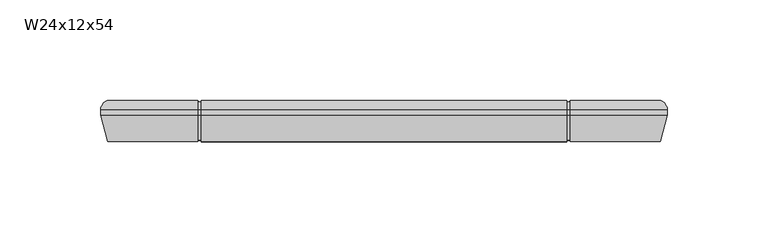
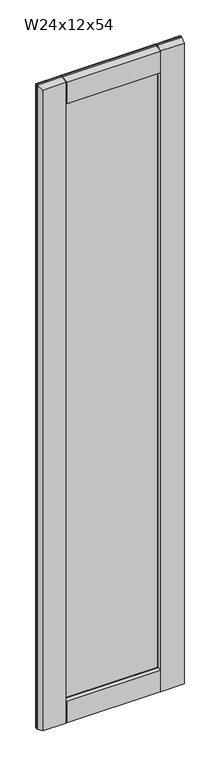
"""IFC4 building model written with IfcOpenShell, lengths in millimetres: furniture geometry, Cabinet-Wall-Merillat-Double_Door-Marlin : W24x12x54."""

from ifc_helpers import new_model, si_unit, frame, origin, place, context, project, spatial, polyline, circle_curve, ellipse_curve, outline, extrude, source, transform, mapped, element, save
from ifc_brep_helpers import plane_surface, cylinder_surface, advanced_brep


def w24x12x54_5feed744(model_context):
    return source(origin(), model_context, "Body", "SolidModel", [
        advanced_brep(
        [(541.0528392, 401.6121, 2108.2), (541.0528392, 401.6121, 787.4), (537.9563467, 406.0825, 790.4964925), (537.9563467, 406.0825, 2105.1035075), (541.0528392, 398.8435, 2108.2), (541.0528392, 398.8435, 787.4), (537.5476392, 385.7625, 2104.6948), (537.5476392, 385.7625, 790.9052), (492.8516765, 385.7625, 2059.9988372), (492.4815448, 386.55625, 2059.6287055), (490.4003857, 391.01931, 2057.5475465), (490.4003857, 391.01931, 838.0524535), (492.4815448, 386.55625, 835.9712945), (492.8516765, 385.7625, 835.6011628), (491.8001552, 393.2594093, 2058.947316), (491.8001552, 393.2594093, 836.652684), (506.1278392, 393.5095, 2073.275), (506.1278392, 393.5095, 822.325), (506.1278392, 398.3355, 2073.275), (506.1278392, 398.3355, 822.325), (491.8001552, 398.5855907, 2058.947316), (491.8001552, 398.5855907, 836.652684), (490.4003857, 400.82569, 2057.5475465), (490.4003857, 400.82569, 838.0524535), (492.4815448, 405.28875, 2059.6287055), (492.848809, 406.0763508, 2059.9959698), (492.8516765, 406.0825, 835.6011628), (492.4815448, 405.28875, 835.9712945), (263.1618317, 406.0825, 790.4964925), (308.2295579, 406.0825, 790.4964925), (308.2295579, 401.6121, 787.4), (260.0653392, 401.6121, 787.4), (492.848809, 401.6121, 787.4), (492.848809, 406.0825, 790.4964925), (491.261309, 401.6121, 787.4), (309.8170579, 401.6121, 787.4), (309.8170579, 406.0825, 790.4964925), (491.261309, 406.0825, 790.4964925), (308.2295579, 398.8435, 787.4), (260.0653392, 398.8435, 787.4), (492.848809, 398.8435, 787.4), (491.261309, 398.8435, 787.4), (309.8170579, 398.8435, 787.4), (308.2295579, 385.7625, 790.9052), (263.5705392, 385.7625, 790.9052), (491.261309, 385.7625, 790.9052), (309.8170579, 385.7625, 790.9052), (492.848809, 385.7625, 790.9052), (310.7177927, 391.01931, 838.0524535), (308.6366337, 386.55625, 835.9712945), (309.8170579, 386.55625, 835.9712945), (309.8170579, 385.7625, 835.6011628), (491.261309, 385.7625, 835.6011628), (491.261309, 386.55625, 835.9712945), (309.3180233, 393.2594093, 836.652684), (294.9903392, 393.5095, 822.325), (294.9903392, 398.3355, 822.325), (309.3180233, 398.5855907, 836.652684), (310.7177927, 400.82569, 838.0524535), (491.261309, 405.28875, 835.9712945), (491.261309, 406.0825, 835.6011628), (309.8170579, 406.0825, 835.6011628), (309.8170579, 405.28875, 835.9712945), (308.6366337, 405.28875, 835.9712945), (260.0653392, 401.6121, 2108.2), (263.1618317, 406.0825, 2105.1035075), (260.0653392, 398.8435, 2108.2), (263.5705392, 385.7625, 2104.6948), (308.266502, 385.7625, 835.6011628), (310.7177927, 391.01931, 2057.5475465), (308.6366337, 386.55625, 2059.6287055), (308.266502, 385.7625, 2059.9988372), (309.3180233, 393.2594093, 2058.947316), (294.9903392, 393.5095, 2073.275), (294.9903392, 398.3355, 2073.275), (309.3180233, 398.5855907, 2058.947316), (310.7177927, 400.82569, 2057.5475465), (308.266502, 406.0825, 835.6011628), (308.266502, 406.0825, 2059.9988372), (308.6366337, 405.28875, 2059.6287055), (492.848809, 406.0825, 2105.1035075), (492.848809, 401.6121, 2108.2), (308.2295579, 401.6121, 2108.2), (308.2295579, 406.0825, 2105.1035075), (309.8170579, 401.6121, 2108.2), (491.261309, 401.6121, 2108.2), (491.261309, 406.0825, 2105.1035075), (309.8170579, 406.0825, 2105.1035075), (492.848809, 398.8435, 2108.2), (308.2295579, 398.8435, 2108.2), (309.8170579, 398.8435, 2108.2), (491.261309, 398.8435, 2108.2), (492.848809, 385.7625, 2104.6948), (308.2295579, 385.7625, 2104.6948), (309.8170579, 385.7625, 2104.6948), (491.261309, 385.7625, 2104.6948), (309.8170579, 385.7625, 2059.9988372), (491.261309, 385.7625, 2059.9988372), (491.261309, 386.55625, 2059.6287055), (309.8170579, 386.55625, 2059.6287055), (309.8170579, 405.28875, 2059.6287055), (309.8170579, 406.0825, 2059.9988372), (491.261309, 406.0825, 2059.9988372), (491.261309, 405.28875, 2059.6287055), (309.8170579, 405.28875, 2104.9526052), (309.8170579, 401.6121, 2107.40625), (309.8170579, 398.9480037, 2107.40625), (309.8170579, 386.55625, 2104.0857412), (308.2295579, 386.55625, 2059.6287055), (308.2295579, 386.55625, 2104.0857412), (308.2295579, 398.9480037, 2107.40625), (308.2295579, 401.6121, 2107.40625), (308.2295579, 405.28875, 2104.9526052), (308.2295579, 405.28875, 2059.6287055), (492.848809, 405.28875, 2059.6287055), (492.848809, 405.28875, 2104.9526052), (492.848809, 401.6121, 2107.40625), (492.848809, 398.9480037, 2107.40625), (492.848809, 386.55625, 2104.0857412), (492.848809, 386.55625, 2059.6287055), (491.261309, 386.55625, 2104.0857412), (491.261309, 398.9480037, 2107.40625), (491.261309, 401.6121, 2107.40625), (491.261309, 405.28875, 2104.9526052), (492.848809, 386.55625, 835.9712945), (492.848809, 386.55625, 791.5142588), (492.848809, 398.9480037, 788.19375), (492.848809, 401.6121, 788.19375), (492.848809, 405.28875, 790.6473948), (492.848809, 405.28875, 835.9712945), (491.261309, 405.28875, 790.6473948), (491.261309, 401.6121, 788.19375), (491.261309, 398.9480037, 788.19375), (491.261309, 386.55625, 791.5142588), (309.8170579, 386.55625, 791.5142588), (309.8170579, 398.9480037, 788.19375), (309.8170579, 401.6121, 788.19375), (309.8170579, 405.28875, 790.6473948), (308.2295579, 405.28875, 835.9712945), (308.2295579, 405.28875, 790.6473948), (308.2295579, 401.6121, 788.19375), (308.2295579, 398.9480037, 788.19375), (308.2295579, 386.55625, 791.5142588), (308.2295579, 386.55625, 835.9712945)],
        [
            (0, 1),
            (1, 2, ellipse_curve(frame((536.2776392, 401.6121, 792.1752), z_axis=(0.7071067811865475, 0.0, 0.7071067811865475), x_axis=(-0.7071067811865474, 0.0, 0.7071067811865476)), 6.7531526, 4.7752)),
            (2, 3),
            (3, 0, ellipse_curve(frame((536.2776392, 401.6121, 2103.4248), z_axis=(0.7071067811865475, 0.0, -0.7071067811865475), x_axis=(0.7071067811865474, 0.0, 0.7071067811865476)), 6.7531526, 4.7752)),
            (0, 4),
            (4, 5),
            (5, 1),
            (4, 6),
            (6, 7),
            (7, 5),
            (8, 9),
            (9, 10),
            (10, 11),
            (11, 12),
            (12, 13),
            (13, 8),
            (10, 14, ellipse_curve(frame((491.8276392, 391.6848492, 2058.9748), z_axis=(0.7071067811865475, 0.0, -0.7071067811865475), x_axis=(0.7071067811865474, 0.0, 0.7071067811865476)), 2.2271035, 1.5748)),
            (14, 15),
            (15, 11, ellipse_curve(frame((491.8276392, 391.6848492, 836.6252), z_axis=(0.7071067811865475, 0.0, 0.7071067811865475), x_axis=(-0.7071067811865474, 0.0, 0.7071067811865476)), 2.2271035, 1.5748)),
            (14, 16),
            (16, 17),
            (17, 15),
            (16, 18),
            (18, 19),
            (19, 17),
            (18, 20),
            (20, 21),
            (21, 19),
            (20, 22, ellipse_curve(frame((491.8276392, 400.1601508, 2058.9748), z_axis=(0.7071067811865475, 0.0, -0.7071067811865475), x_axis=(0.7071067811865474, 0.0, 0.7071067811865476)), 2.2271035, 1.5748)),
            (22, 23),
            (23, 21, ellipse_curve(frame((491.8276392, 400.1601508, 836.6252), z_axis=(0.7071067811865475, 0.0, 0.7071067811865475), x_axis=(-0.7071067811865474, 0.0, 0.7071067811865476)), 2.2271035, 1.5748)),
            (22, 24),
            (24, 25),
            (25, 26),
            (26, 27),
            (27, 23),
            (28, 29),
            (29, 30, circle_curve(frame((308.2295579, 401.6121, 792.1752), z_axis=(-1.0, 0.0, 0.0), x_axis=(0.0, -1.0, 0.0)), 4.7752)),
            (30, 31),
            (31, 28, ellipse_curve(frame((264.8405392, 401.6121, 792.1752), z_axis=(0.7071067811865475, 0.0, -0.7071067811865475), x_axis=(0.7071067811865476, 0.0, 0.7071067811865474)), 6.7531526, 4.7752)),
            (1, 32),
            (32, 33, circle_curve(frame((492.848809, 401.6121, 792.1752), z_axis=(1.0, 0.0, 0.0), x_axis=(0.0, -1.0, 0.0)), 4.7752)),
            (33, 2),
            (34, 35),
            (35, 36, circle_curve(frame((309.8170579, 401.6121, 792.1752), z_axis=(1.0, 0.0, 0.0), x_axis=(0.0, -1.0, 0.0)), 4.7752)),
            (36, 37),
            (37, 34, circle_curve(frame((491.261309, 401.6121, 792.1752), z_axis=(-1.0, 0.0, 0.0), x_axis=(0.0, -1.0, 0.0)), 4.7752)),
            (30, 38),
            (38, 39),
            (39, 31),
            (5, 40),
            (40, 32),
            (41, 42),
            (42, 35),
            (34, 41),
            (38, 43),
            (43, 44),
            (44, 39),
            (45, 46),
            (46, 42),
            (41, 45),
            (7, 47),
            (47, 40),
            (48, 49),
            (49, 50),
            (50, 51),
            (51, 52),
            (52, 53),
            (53, 12),
            (11, 48),
            (15, 54),
            (54, 48, ellipse_curve(frame((309.2905392, 391.6848492, 836.6252), z_axis=(0.7071067811865475, 0.0, -0.7071067811865475), x_axis=(0.7071067811865476, 0.0, 0.7071067811865474)), 2.2271035, 1.5748)),
            (17, 55),
            (55, 54),
            (19, 56),
            (56, 55),
            (21, 57),
            (57, 56),
            (23, 58),
            (58, 57, ellipse_curve(frame((309.2905392, 400.1601508, 836.6252), z_axis=(0.7071067811865475, 0.0, -0.7071067811865475), x_axis=(0.7071067811865476, 0.0, 0.7071067811865474)), 2.2271035, 1.5748)),
            (27, 59),
            (59, 60),
            (60, 61),
            (61, 62),
            (62, 63),
            (63, 58),
            (31, 64),
            (64, 65, ellipse_curve(frame((264.8405392, 401.6121, 2103.4248), z_axis=(-0.7071067811865475, 0.0, -0.7071067811865475), x_axis=(0.7071067811865474, 0.0, -0.7071067811865476)), 6.7531526, 4.7752)),
            (65, 28),
            (39, 66),
            (66, 64),
            (44, 67),
            (67, 66),
            (68, 49),
            (48, 69),
            (69, 70),
            (70, 71),
            (71, 68),
            (54, 72),
            (72, 69, ellipse_curve(frame((309.2905392, 391.6848492, 2058.9748), z_axis=(-0.7071067811865475, 0.0, -0.7071067811865475), x_axis=(0.7071067811865474, 0.0, -0.7071067811865476)), 2.2271035, 1.5748)),
            (55, 73),
            (73, 72),
            (56, 74),
            (74, 73),
            (57, 75),
            (75, 74),
            (58, 76),
            (76, 75, ellipse_curve(frame((309.2905392, 400.1601508, 2058.9748), z_axis=(-0.7071067811865475, 0.0, -0.7071067811865475), x_axis=(0.7071067811865474, 0.0, -0.7071067811865476)), 2.2271035, 1.5748)),
            (63, 77),
            (77, 78),
            (78, 79),
            (79, 76),
            (3, 80),
            (80, 81, circle_curve(frame((492.848809, 401.6121, 2103.4248), z_axis=(1.0, 0.0, 0.0), x_axis=(0.0, -1.0, 0.0)), 4.7752)),
            (81, 0),
            (64, 82),
            (82, 83, circle_curve(frame((308.2295579, 401.6121, 2103.4248), z_axis=(-1.0, 0.0, 0.0), x_axis=(0.0, -1.0, 0.0)), 4.7752)),
            (83, 65),
            (84, 85),
            (85, 86, circle_curve(frame((491.261309, 401.6121, 2103.4248), z_axis=(-1.0, 0.0, 0.0), x_axis=(0.0, -1.0, 0.0)), 4.7752)),
            (86, 87),
            (87, 84, circle_curve(frame((309.8170579, 401.6121, 2103.4248), z_axis=(1.0, 0.0, 0.0), x_axis=(0.0, -1.0, 0.0)), 4.7752)),
            (81, 88),
            (88, 4),
            (66, 89),
            (89, 82),
            (90, 91),
            (91, 85),
            (84, 90),
            (88, 92),
            (92, 6),
            (67, 93),
            (93, 89),
            (94, 95),
            (95, 91),
            (90, 94),
            (51, 46),
            (45, 52),
            (43, 68),
            (71, 93),
            (92, 8),
            (13, 47),
            (96, 97),
            (97, 95),
            (94, 96),
            (9, 98),
            (98, 97),
            (96, 99),
            (99, 70),
            (69, 10),
            (72, 14),
            (73, 16),
            (74, 18),
            (75, 20),
            (76, 22),
            (79, 100),
            (100, 101),
            (101, 102),
            (102, 103),
            (103, 24),
            (33, 26),
            (25, 80),
            (36, 61),
            (60, 37),
            (83, 78),
            (77, 29),
            (86, 102),
            (101, 87),
            (100, 104),
            (104, 105, circle_curve(frame((309.8170579, 401.6121, 2103.4248), z_axis=(1.0, 0.0, 0.0), x_axis=(0.0, 0.0, 1.0)), 3.98145)),
            (105, 106),
            (106, 107),
            (107, 99),
            (71, 108),
            (108, 109),
            (109, 110),
            (110, 111),
            (111, 112, circle_curve(frame((308.2295579, 401.6121, 2103.4248), z_axis=(-1.0, 0.0, 0.0), x_axis=(0.0, 0.0, 1.0)), 3.98145)),
            (112, 113),
            (113, 78),
            (113, 79),
            (112, 104),
            (111, 105),
            (110, 106),
            (109, 107),
            (108, 70),
            (25, 114),
            (114, 115),
            (115, 116, circle_curve(frame((492.848809, 401.6121, 2103.4248), z_axis=(1.0, 0.0, 0.0), x_axis=(0.0, 0.0, 1.0)), 3.98145)),
            (116, 117),
            (117, 118),
            (118, 119),
            (119, 8),
            (98, 120),
            (120, 121),
            (121, 122),
            (122, 123, circle_curve(frame((491.261309, 401.6121, 2103.4248), z_axis=(-1.0, 0.0, 0.0), x_axis=(0.0, 0.0, 1.0)), 3.98145)),
            (123, 103),
            (24, 114),
            (123, 115),
            (122, 116),
            (121, 117),
            (120, 118),
            (9, 119),
            (13, 124),
            (124, 125),
            (125, 126),
            (126, 127),
            (127, 128, circle_curve(frame((492.848809, 401.6121, 792.1752), z_axis=(1.0, 0.0, 0.0), x_axis=(0.0, 0.0, 1.0)), 3.98145)),
            (128, 129),
            (129, 26),
            (59, 130),
            (130, 131, circle_curve(frame((491.261309, 401.6121, 792.1752), z_axis=(-1.0, 0.0, 0.0), x_axis=(0.0, 0.0, 1.0)), 3.98145)),
            (131, 132),
            (132, 133),
            (133, 53),
            (12, 124),
            (133, 125),
            (132, 126),
            (131, 127),
            (130, 128),
            (27, 129),
            (50, 134),
            (134, 135),
            (135, 136),
            (136, 137, circle_curve(frame((309.8170579, 401.6121, 792.1752), z_axis=(1.0, 0.0, 0.0), x_axis=(0.0, 0.0, 1.0)), 3.98145)),
            (137, 62),
            (138, 139),
            (139, 140, circle_curve(frame((308.2295579, 401.6121, 792.1752), z_axis=(-1.0, 0.0, 0.0), x_axis=(0.0, 0.0, 1.0)), 3.98145)),
            (140, 141),
            (141, 142),
            (142, 143),
            (143, 68),
            (77, 138),
            (63, 138),
            (143, 49),
            (142, 134),
            (141, 135),
            (140, 136),
            (139, 137),
        ],
        [
            cylinder_surface(frame((536.2776392, 401.6121, 2108.2), z_axis=(0.0, 0.0, 1.0), x_axis=(0.0, -1.0, 0.0)), 4.7752),
            plane_surface(frame((541.0528392, 401.6121, 2108.2), z_axis=(1.0, 0.0, 0.0), x_axis=(0.0, 0.0, -1.0))),
            plane_surface(frame((541.0528392, 398.8435, 2108.2), z_axis=(0.9659229350723619, -0.25882983502910506, 0.0), x_axis=(0.0, 0.0, -1.0))),
            plane_surface(frame((492.8516765, 385.7625, 2059.9988372), z_axis=(-0.9063077870366099, -0.4226182617407856, 0.0), x_axis=(0.0, 0.0, -1.0))),
            cylinder_surface(frame((491.8276392, 391.6848492, 2108.2), z_axis=(0.0, 0.0, 1.0000000000000002), x_axis=(-0.01745240643729364, 0.9998476951563912, 0.0)), 1.5748),
            plane_surface(frame((491.8001552, 393.2594093, 2058.947316), z_axis=(-0.017452406437322144, 0.9998476951563906, 0.0), x_axis=(0.0, 0.0, -1.0))),
            plane_surface(frame((506.1278392, 393.5095, 2073.275), z_axis=(-1.0, 0.0, 0.0), x_axis=(0.0, 0.0, -1.0))),
            plane_surface(frame((506.1278392, 398.3355, 2073.275), z_axis=(-0.01745240643727848, -0.9998476951563914, 0.0), x_axis=(0.0, 0.0, -1.0))),
            cylinder_surface(frame((491.8276392, 400.1601508, 2108.2), z_axis=(0.0, 0.0, 1.0000000000000002), x_axis=(-0.9063077870367326, 0.42261826174052236, 0.0)), 1.5748),
            plane_surface(frame((490.4003857, 400.82569, 2057.5475465), z_axis=(-0.9063077870366333, 0.4226182617407352, 0.0), x_axis=(0.0, 0.0, -1.0))),
            cylinder_surface(frame((541.0528392, 401.6121, 792.1752), z_axis=(1.0, 0.0, 0.0), x_axis=(0.0, -1.0, 0.0)), 4.7752),
            plane_surface(frame((541.0528392, 401.6121, 787.4), z_axis=(0.0, 0.0, -1.0), x_axis=(-1.0, 0.0, 0.0))),
            plane_surface(frame((541.0528392, 398.8435, 787.4), z_axis=(0.0, -0.2588298350291095, -0.9659229350723607), x_axis=(-1.0, 0.0, 0.0))),
            plane_surface(frame((492.8516765, 385.7625, 835.6011628), z_axis=(0.0, -0.42261826174078143, 0.9063077870366119), x_axis=(-1.0, 0.0, 0.0))),
            cylinder_surface(frame((541.0528392, 391.6848492, 836.6252), z_axis=(1.0000000000000002, 0.0, 0.0), x_axis=(0.0, 0.9998476951563913, 0.017452406437289025)), 1.5748),
            plane_surface(frame((491.8001552, 393.2594093, 836.652684), z_axis=(0.0, 0.9998476951563907, 0.01745240643731753), x_axis=(-1.0, 0.0, 0.0))),
            plane_surface(frame((506.1278392, 393.5095, 822.325), z_axis=(0.0, 0.0, 1.0), x_axis=(-1.0, 0.0, 0.0))),
            plane_surface(frame((506.1278392, 398.3355, 822.325), z_axis=(0.0, -0.9998476951563913, 0.017452406437283095), x_axis=(-1.0, 0.0, 0.0))),
            cylinder_surface(frame((541.0528392, 400.1601508, 836.6252), z_axis=(1.0000000000000002, 0.0, 0.0), x_axis=(0.0, 0.4226182617405265, 0.9063077870367306)), 1.5748),
            plane_surface(frame((490.4003857, 400.82569, 838.0524535), z_axis=(0.0, 0.4226182617407394, 0.9063077870366314), x_axis=(-1.0, 0.0, 0.0))),
            cylinder_surface(frame((264.8405392, 401.6121, 787.4), z_axis=(0.0, 0.0, -1.0), x_axis=(0.0, -1.0, 0.0)), 4.7752),
            plane_surface(frame((260.0653392, 401.6121, 787.4), z_axis=(-1.0, 0.0, 0.0), x_axis=(0.0, 0.0, 1.0))),
            plane_surface(frame((260.0653392, 398.8435, 787.4), z_axis=(-0.9659229350723619, -0.25882983502910506, 0.0), x_axis=(0.0, 0.0, 1.0))),
            plane_surface(frame((308.266502, 385.7625, 835.6011628), z_axis=(0.9063077870366099, -0.4226182617407856, 0.0), x_axis=(0.0, 0.0, 1.0))),
            cylinder_surface(frame((309.2905392, 391.6848492, 787.4), z_axis=(0.0, 0.0, -1.0000000000000002), x_axis=(0.01745240643729364, 0.9998476951563912, 0.0)), 1.5748),
            plane_surface(frame((309.3180233, 393.2594093, 836.652684), z_axis=(0.017452406437322144, 0.9998476951563906, 0.0), x_axis=(0.0, 0.0, 1.0))),
            plane_surface(frame((294.9903392, 393.5095, 822.325), z_axis=(1.0, 0.0, 0.0), x_axis=(0.0, 0.0, 1.0))),
            plane_surface(frame((294.9903392, 398.3355, 822.325), z_axis=(0.01745240643727848, -0.9998476951563914, 0.0), x_axis=(0.0, 0.0, 1.0))),
            cylinder_surface(frame((309.2905392, 400.1601508, 787.4), z_axis=(0.0, 0.0, -1.0000000000000002), x_axis=(0.9063077870367326, 0.42261826174052236, 0.0)), 1.5748),
            plane_surface(frame((310.7177927, 400.82569, 838.0524535), z_axis=(0.9063077870366333, 0.4226182617407352, 0.0), x_axis=(0.0, 0.0, 1.0))),
            cylinder_surface(frame((260.0653392, 401.6121, 2103.4248), z_axis=(-1.0, 0.0, 0.0), x_axis=(0.0, -1.0, 0.0)), 4.7752),
            plane_surface(frame((260.0653392, 401.6121, 2108.2), z_axis=(0.0, 0.0, 1.0), x_axis=(1.0, 0.0, 0.0))),
            plane_surface(frame((260.0653392, 398.8435, 2108.2), z_axis=(0.0, -0.2588298350291006, 0.9659229350723632), x_axis=(1.0, 0.0, 0.0))),
            plane_surface(frame((263.5705392, 385.7625, 2104.6948), z_axis=(0.0, -1.0, 0.0), x_axis=(1.0, 0.0, 0.0))),
            plane_surface(frame((308.266502, 385.7625, 2059.9988372), z_axis=(0.0, -0.42261826174078976, -0.9063077870366079), x_axis=(1.0, 0.0, 0.0))),
            cylinder_surface(frame((260.0653392, 391.6848492, 2058.9748), z_axis=(-1.0000000000000002, 0.0, 0.0), x_axis=(0.0, 0.999847695156391, -0.017452406437298253)), 1.5748),
            plane_surface(frame((309.3180233, 393.2594093, 2058.947316), z_axis=(0.0, 0.9998476951563905, -0.01745240643732676), x_axis=(1.0, 0.0, 0.0))),
            plane_surface(frame((294.9903392, 393.5095, 2073.275), z_axis=(0.0, 0.0, -1.0), x_axis=(1.0, 0.0, 0.0))),
            plane_surface(frame((294.9903392, 398.3355, 2073.275), z_axis=(0.0, -0.9998476951563915, -0.017452406437273867), x_axis=(1.0, 0.0, 0.0))),
            cylinder_surface(frame((260.0653392, 400.1601508, 2058.9748), z_axis=(-1.0000000000000002, 0.0, 0.0), x_axis=(0.0, 0.4226182617405182, -0.9063077870367346)), 1.5748),
            plane_surface(frame((310.7177927, 400.82569, 2057.5475465), z_axis=(0.0, 0.422618261740731, -0.9063077870366353), x_axis=(1.0, 0.0, 0.0))),
            plane_surface(frame((308.266502, 406.0825, 2059.9988372), z_axis=(0.0, 1.0, 0.0), x_axis=(1.0, 0.0, 0.0))),
            plane_surface(frame((309.8170579, 406.0825, 2059.9988372), z_axis=(-1.0000000000000002, 0.0, 0.0), x_axis=(0.0, -0.9063077870366177, -0.4226182617407689))),
            plane_surface(frame((308.2295579, 406.0825, 2059.9988372), z_axis=(1.0000000000000002, 0.0, 0.0), x_axis=(0.0, 0.9063077870366177, 0.4226182617407689))),
            plane_surface(frame((309.8170579, 406.0825, 2059.9988372), z_axis=(0.0, -0.4226182617407689, 0.9063077870366177), x_axis=(-1.0, 0.0, 0.0))),
            plane_surface(frame((309.8170579, 405.28875, 2059.6287055), z_axis=(0.0, 1.0, 0.0), x_axis=(-1.0, 0.0, 0.0))),
            cylinder_surface(frame((308.2295579, 401.6121, 2103.4248), z_axis=(-1.0, 0.0, 0.0), x_axis=(0.0, 0.0, 1.0)), 3.98145),
            plane_surface(frame((309.8170579, 401.6121, 2107.40625), z_axis=(0.0, 0.0, 1.0), x_axis=(-1.0, 0.0, 0.0))),
            plane_surface(frame((309.8170579, 398.9480037, 2107.40625), z_axis=(0.0, -0.2588298350291571, 0.965922935072348), x_axis=(-1.0, 0.0, 0.0))),
            plane_surface(frame((309.8170579, 386.55625, 2104.0857412), z_axis=(0.0, -1.0, 0.0), x_axis=(-1.0, 0.0, 0.0))),
            plane_surface(frame((309.8170579, 386.55625, 2059.6287055), z_axis=(0.0, 0.4226182617408151, 0.906307787036596), x_axis=(-1.0, 0.0, 0.0))),
            plane_surface(frame((492.848809, 406.0825, 2059.9988372), z_axis=(-1.0, 0.0, 0.0), x_axis=(0.0, -0.9063077870366254, -0.42261826174075223))),
            plane_surface(frame((491.261309, 406.0825, 2059.9988372), z_axis=(1.0, 0.0, 0.0), x_axis=(0.0, 0.9063077870366254, 0.42261826174075223))),
            plane_surface(frame((492.848809, 406.0825, 2059.9988372), z_axis=(0.0, -0.42261826174075223, 0.9063077870366254), x_axis=(-1.0, 0.0, 0.0))),
            plane_surface(frame((492.848809, 405.28875, 2059.6287055), z_axis=(0.0, 1.0, 0.0), x_axis=(-1.0, 0.0, 0.0))),
            cylinder_surface(frame((491.261309, 401.6121, 2103.4248), z_axis=(-1.0, 0.0, 0.0), x_axis=(0.0, 0.0, 1.0)), 3.98145),
            plane_surface(frame((492.848809, 401.6121, 2107.40625), z_axis=(0.0, 0.0, 1.0), x_axis=(-1.0, 0.0, 0.0))),
            plane_surface(frame((492.848809, 398.9480037, 2107.40625), z_axis=(0.0, -0.258829835029159, 0.9659229350723475), x_axis=(-1.0, 0.0, 0.0))),
            plane_surface(frame((492.848809, 386.55625, 2104.0857412), z_axis=(0.0, -1.0, 0.0), x_axis=(-1.0, 0.0, 0.0))),
            plane_surface(frame((492.848809, 386.55625, 2059.6287055), z_axis=(0.0, 0.4226182617408322, 0.9063077870365881), x_axis=(-1.0, 0.0, 0.0))),
            plane_surface(frame((492.848809, 401.6121, 796.9504), z_axis=(-1.0, 0.0, 0.0), x_axis=(0.0, 1.0, 0.0))),
            plane_surface(frame((491.261309, 401.6121, 796.9504), z_axis=(1.0, 0.0, 0.0), x_axis=(0.0, -1.0, 0.0))),
            plane_surface(frame((492.848809, 385.7625, 835.6011628), z_axis=(0.0, 0.4226182617407559, -0.9063077870366237), x_axis=(-1.0, 0.0, 0.0))),
            plane_surface(frame((492.848809, 386.55625, 835.9712945), z_axis=(0.0, -1.0, 0.0), x_axis=(-1.0, 0.0, 0.0))),
            plane_surface(frame((492.848809, 386.55625, 791.5142588), z_axis=(0.0, -0.25882983502944146, -0.9659229350722718), x_axis=(-1.0, 0.0, 0.0))),
            plane_surface(frame((492.848809, 398.9480037, 788.19375), z_axis=(0.0, 0.0, -1.0), x_axis=(-1.0, 0.0, 0.0))),
            cylinder_surface(frame((491.261309, 401.6121, 792.1752), z_axis=(-1.0, 0.0, 0.0), x_axis=(0.0, 0.0, 1.0)), 3.98145),
            plane_surface(frame((492.848809, 405.28875, 790.6473948), z_axis=(0.0, 1.0, 0.0), x_axis=(-1.0, 0.0, 0.0))),
            plane_surface(frame((492.848809, 405.28875, 835.9712945), z_axis=(0.0, -0.42261826174073325, -0.9063077870366342), x_axis=(-1.0, 0.0, 0.0))),
            plane_surface(frame((309.8170579, 405.28875, 835.9712945), z_axis=(-1.0, 0.0, 0.0), x_axis=(0.0, 0.9063077870366539, -0.42261826174069095))),
            plane_surface(frame((308.2295579, 405.28875, 835.9712945), z_axis=(1.0, 0.0, 0.0), x_axis=(0.0, -0.9063077870366539, 0.42261826174069095))),
            plane_surface(frame((309.8170579, 405.28875, 835.9712945), z_axis=(0.0, -0.42261826174069095, -0.9063077870366539), x_axis=(-1.0, 0.0, 0.0))),
            plane_surface(frame((309.8170579, 385.7625, 835.6011628), z_axis=(0.0, 0.42261826174079387, -0.9063077870366061), x_axis=(-1.0, 0.0, 0.0))),
            plane_surface(frame((309.8170579, 386.55625, 835.9712945), z_axis=(0.0, -1.0, 0.0), x_axis=(-1.0, 0.0, 0.0))),
            plane_surface(frame((309.8170579, 386.55625, 791.5142588), z_axis=(0.0, -0.25882983502944, -0.9659229350722722), x_axis=(-1.0, 0.0, 0.0))),
            plane_surface(frame((309.8170579, 398.9480037, 788.19375), z_axis=(0.0, 0.0, -1.0), x_axis=(-1.0, 0.0, 0.0))),
            cylinder_surface(frame((308.2295579, 401.6121, 792.1752), z_axis=(-1.0, 0.0, 0.0), x_axis=(0.0, 0.0, 1.0)), 3.98145),
            plane_surface(frame((309.8170579, 405.28875, 790.6473948), z_axis=(0.0, 1.0, 0.0), x_axis=(-1.0, 0.0, 0.0))),
        ],
        [
            (0, [[1, 2, 3, 4]]),
            (1, [[5, 6, 7, -1]]),
            (2, [[8, 9, 10, -6]]),
            (3, [[11, 12, 13, 14, 15, 16]]),
            (4, [[17, 18, 19, -13]]),
            (5, [[20, 21, 22, -18]]),
            (6, [[23, 24, 25, -21]]),
            (7, [[26, 27, 28, -24]]),
            (8, [[29, 30, 31, -27]]),
            (9, [[32, 33, 34, 35, 36, -30]]),
            (10, [[37, 38, 39, 40]]),
            (10, [[41, 42, 43, -2]]),
            (10, [[44, 45, 46, 47]]),
            (11, [[-39, 48, 49, 50]]),
            (11, [[51, 52, -41, -7]]),
            (11, [[53, 54, -44, 55]]),
            (12, [[-49, 56, 57, 58]]),
            (12, [[59, 60, -53, 61]]),
            (12, [[62, 63, -51, -10]]),
            (13, [[64, 65, 66, 67, 68, 69, -14, 70]]),
            (14, [[71, 72, -70, -19]]),
            (15, [[73, 74, -71, -22]]),
            (16, [[75, 76, -73, -25]]),
            (17, [[77, 78, -75, -28]]),
            (18, [[79, 80, -77, -31]]),
            (19, [[-36, 81, 82, 83, 84, 85, 86, -79]]),
            (20, [[87, 88, 89, -40]]),
            (21, [[90, 91, -87, -50]]),
            (22, [[92, 93, -90, -58]]),
            (23, [[94, -64, 95, 96, 97, 98]]),
            (24, [[99, 100, -95, -72]]),
            (25, [[101, 102, -99, -74]]),
            (26, [[103, 104, -101, -76]]),
            (27, [[105, 106, -103, -78]]),
            (28, [[107, 108, -105, -80]]),
            (29, [[-86, 109, 110, 111, 112, -107]]),
            (30, [[113, 114, 115, -4]]),
            (30, [[116, 117, 118, -88]]),
            (30, [[119, 120, 121, 122]]),
            (31, [[-115, 123, 124, -5]]),
            (31, [[125, 126, -116, -91]]),
            (31, [[127, 128, -119, 129]]),
            (32, [[-124, 130, 131, -8]]),
            (32, [[132, 133, -125, -93]]),
            (32, [[134, 135, -127, 136]]),
            (33, [[-67, 137, -59, 138]]),
            (33, [[-57, 139, -98, 140, -132, -92]]),
            (33, [[-131, 141, -16, 142, -62, -9]]),
            (33, [[143, 144, -134, 145]]),
            (34, [[-12, 146, 147, -143, 148, 149, -96, 150]]),
            (35, [[-150, -100, 151, -17]]),
            (36, [[-151, -102, 152, -20]]),
            (37, [[-152, -104, 153, -23]]),
            (38, [[-153, -106, 154, -26]]),
            (39, [[-154, -108, 155, -29]]),
            (40, [[-112, 156, 157, 158, 159, 160, -32, -155]]),
            (41, [[-43, 161, -34, 162, -113, -3]]),
            (41, [[-46, 163, -83, 164]]),
            (41, [[-118, 165, -110, 166, -37, -89]]),
            (41, [[-121, 167, -158, 168]]),
            (42, [[-148, -145, -136, -129, -122, -168, -157, 169, 170, 171, 172, 173]]),
            (43, [[-165, -117, -126, -133, -140, 174, 175, 176, 177, 178, 179, 180]]),
            (44, [[181, -111, -180]]),
            (45, [[-156, -181, -179, 182, -169]]),
            (46, [[-182, -178, 183, -170]]),
            (47, [[-183, -177, 184, -171]]),
            (48, [[-184, -176, 185, -172]]),
            (49, [[-185, -175, 186, -149, -173]]),
            (50, [[-97, -186, -174]]),
            (51, [[-141, -130, -123, -114, -162, 187, 188, 189, 190, 191, 192, 193]]),
            (52, [[-159, -167, -120, -128, -135, -144, -147, 194, 195, 196, 197, 198]]),
            (53, [[-33, 199, -187]]),
            (54, [[-199, -160, -198, 200, -188]]),
            (55, [[-200, -197, 201, -189]]),
            (56, [[-201, -196, 202, -190]]),
            (57, [[-202, -195, 203, -191]]),
            (58, [[-203, -194, -146, 204, -192]]),
            (59, [[-204, -11, -193]]),
            (60, [[-161, -42, -52, -63, -142, 205, 206, 207, 208, 209, 210, 211]]),
            (61, [[-68, -138, -61, -55, -47, -164, -82, 212, 213, 214, 215, 216]]),
            (62, [[-15, 217, -205]]),
            (63, [[-217, -69, -216, 218, -206]]),
            (64, [[-218, -215, 219, -207]]),
            (65, [[-219, -214, 220, -208]]),
            (66, [[-220, -213, 221, -209]]),
            (67, [[-221, -212, -81, 222, -210]]),
            (68, [[-222, -35, -211]]),
            (69, [[-84, -163, -45, -54, -60, -137, -66, 223, 224, 225, 226, 227]]),
            (70, [[228, 229, 230, 231, 232, 233, -139, -56, -48, -38, -166, 234]]),
            (71, [[-109, 235, -234]]),
            (72, [[236, -94, -233]]),
            (73, [[-65, -236, -232, 237, -223]]),
            (74, [[-237, -231, 238, -224]]),
            (75, [[-238, -230, 239, -225]]),
            (76, [[-239, -229, 240, -226]]),
            (77, [[-240, -228, -235, -85, -227]]),
        ],
    ),
        extrude(outline(polyline([(294.9903392, 398.3355), (506.1278392, 398.3355), (506.1278392, 393.5095), (294.9903392, 393.5095), (294.9903392, 398.3355)])), frame((0.0, 0.0, 822.325), z_axis=(0.0, 0.0, 1.0), x_axis=(1.0, 0.0, 0.0)), (0.0, 0.0, 1.0), 1250.95),
    ])


if __name__ == "__main__":
    model = new_model("IFC4")
    model_context = context("Model", 3, world=origin())
    ifc_project = project(units=[si_unit("LENGTHUNIT", "METRE", prefix="MILLI")], contexts=[model_context])
    site = spatial("IfcSite", under=ifc_project)
    building = spatial("IfcBuilding", under=site)
    placement = place(None, origin())
    w24x12x54_shape = w24x12x54_5feed744(model_context)
    element("IfcFurniture", 1, ObjectType="Cabinet-Wall-Merillat-Double_Door-Marlin : W24x12x54", at=placement, inside=building, context=model_context, shape_type="MappedRepresentation", body=[
        mapped(w24x12x54_shape, transform((0.0, 0.0, 0.0), x_axis=(1.0, 0.0, 0.0), y_axis=(0.0, 1.0, 0.0), z_axis=(0.0, 0.0, 1.0))),
    ])
    save(model, "model.ifc")

# Revit data of these elements
# Type "Cabinet-Wall-Merillat-Double_Door-Marlin : W24x12x54"
#   URL = "https://www.merillat.com/"
#   Product Page URL = "https://www.merillat.com/our-products/"
#   Product Line = "Express"
#   Product Group = "Wall Cabinet"
#   Product Documentation Link = "http://merillatbusiness.com/wp-content/uploads/2014/07/Merillat_Classic_Catalog.pdf"
#   Model = "W2442B"
#   Manufacturer = "Merillat"
#   Height Note = "Actual Height of 21 inches Cabinet is 20 1/2 inches"
#   Glass Door Note = "Glass Cabinet doors are only available in specific sizes. Please refer to the catalog for this information before requesting a glass size."
#   Finish = "Wood"
#   Description = "Wall 2442 Butt Door"
#   Construction Type = "Wall Cabinet"
#   Cabinet Construction Note = "Cabinets with B suffix have BUTT doors without a center frame stile:"
#   Assembly Code = "C1030410"
#   Spacing = 0' - 1"
#   Shelving Height = 1' - 0 3/4"
#   Door Spacing = 0' - 0 1/8"
#   Cabinet Door Width = 0' - 11 1/16"
#   Cabinet Door Height = 4' - 4"
#   Depth = 1' - 0"
#   Height = 4' - 6"
#   Top Of Cabinet = 7' - 0"
#   Width = 2' - 0"
#   COBie.Type = no
#   Top and Bottom Visibility = yes
#   Partial Overlay Butt = yes
#   Partial Overlay = no
#   Number of Shelves Greater than one = 3
#   Number of Shelves = 3
#   Middle Shelf = yes
#   Full Overlay Butt = no
#   Full Overlay = no
#   Elevation Swing Line = yes
#   Door Drawer Material = Wood - Merillat - Pecan(1)
#   Cabinet Material = Wood - Merillat - Pecan(1)
#   Cabinet Door Style = element 806847
# Element 1 (IfcFurniture, "Cabinet-Wall-Merillat-Double_Door-Marlin : W24x12x54")
#   Materials on its faces: "Wood - Merillat - Pecan(1)"
# Materials
#   "Wood - Merillat - Pecan(1)": class "Wood", colour RGB 108 67 43, transparency 0, Cost = 0
